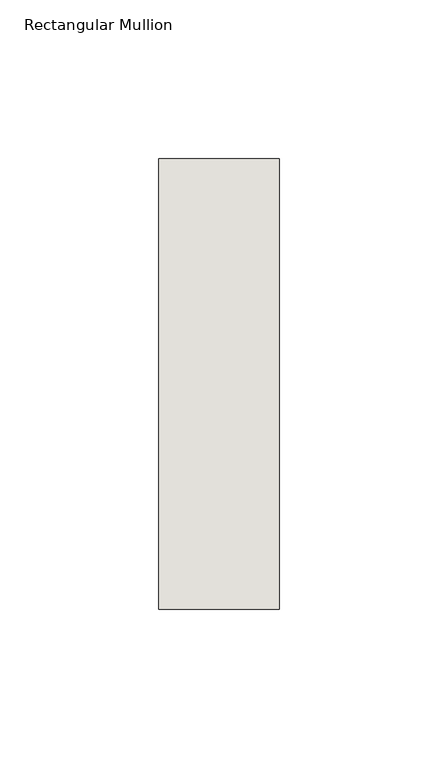
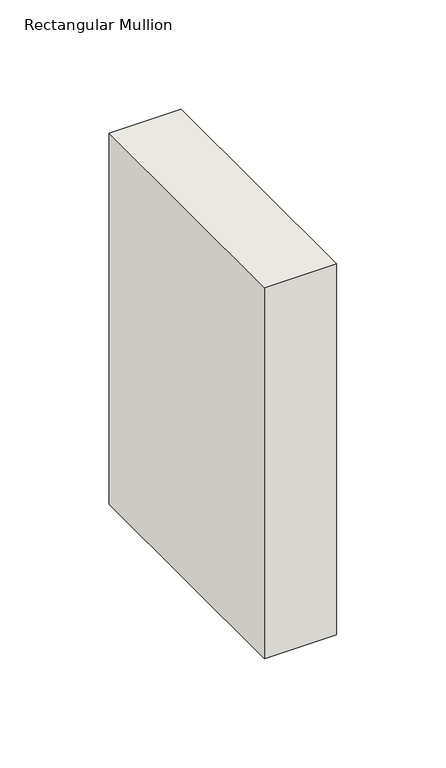
"""IFC4 building model written with IfcOpenShell, lengths in millimetres: wall geometry, Rectangular Mullion : NLRS_21_CWM_hsb-regel 38x142_gen_rsf."""

from ifc_helpers import new_model, si_unit, frame, origin, place, context, project, spatial, polyline, outline, extrude, source, transform, mapped, element, save


def rectangular_mullion_ed461cf7(model_context):
    return source(origin(), model_context, "Body", "SweptSolid", [
        extrude(outline(polyline([(0.0, -71.0), (-38.0, -71.0), (-38.0, 71.0), (0.0, 71.0), (0.0, -71.0)])), frame((0.0, 0.0, -207.0000003), z_axis=(0.0, 0.0, 1.0), x_axis=(1.0, 0.0, 0.0)), (0.0, 0.0, 1.0), 207.0000003),
    ])


if __name__ == "__main__":
    model = new_model("IFC4")
    model_context = context("Model", 3, world=origin())
    ifc_project = project(units=[si_unit("LENGTHUNIT", "METRE", prefix="MILLI")], contexts=[model_context])
    site = spatial("IfcSite", under=ifc_project)
    building = spatial("IfcBuilding", under=site)
    placement = place(None, origin())
    rectangular_mullion_shape = rectangular_mullion_ed461cf7(model_context)
    element("IfcWall", 1, ObjectType="Rectangular Mullion : NLRS_21_CWM_hsb-regel 38x142_gen_rsf", at=placement, inside=building, context=model_context, shape_type="MappedRepresentation", body=[
        mapped(rectangular_mullion_shape, transform((0.0, 0.0, 0.0), x_axis=(1.0, 0.0, 0.0), y_axis=(0.0, 1.0, 0.0), z_axis=(0.0, 0.0, 1.0))),
    ])
    save(model, "model.ifc")

# Revit data of these elements
# Type "Rectangular Mullion : NLRS_21_CWM_hsb-regel 38x142_gen_rsf"
#   Type IfcGUID = "07M7mRoiH1CR8m_RSKIwpF"
#   Assembly Code = "21.10"
#   IfcExportAs = "IfcWall"
#   built-in parameter 1007322 = 0.465879 (stored number, unit not read)
#   built-in parameter 1007321 = 0.062336 (stored number, unit not read)
#   built-in parameter 1007320 = 0.062336 (stored number, unit not read)
# Element 1 (IfcWall, "Rectangular Mullion : NLRS_21_CWM_hsb-regel 38x142_gen_rsf")
#   Materials on its faces: "NLRS_i2_hout naaldhout vuren_gen_rsf"
# Materials
#   "NLRS_i2_hout naaldhout vuren_gen_rsf": class "I - Hout", colour RGB 234 199 147, transparency 0, Keynote = "i2", Manufacturer = "Revit Standards Foundation", URL = "www.revitstandards.org", Description = "hout vuren", Cost = 0
